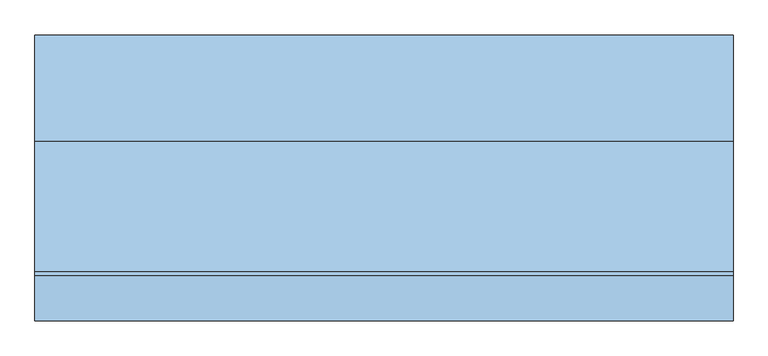
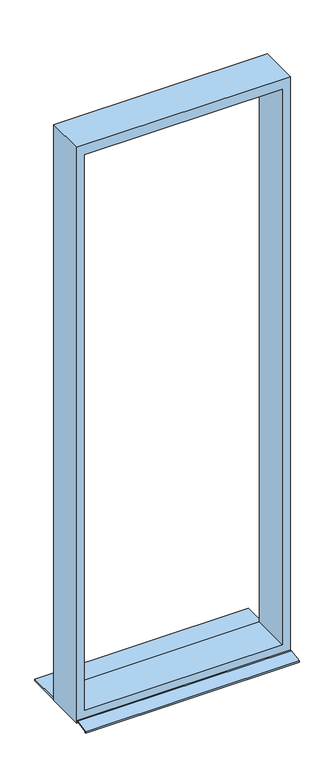
"""IFC4 building model written with IfcOpenShell, lengths in millimetres: window geometry, Fenster - Festverglasung : Feste Verglasung 4.58 x 1.61 2."""

from ifc_helpers import new_model, si_unit, frame, origin, place, context, project, spatial, polyline, outline, extrude, source, transform, mapped, element, save


def window_990d40f6(model_context):
    return source(origin(), model_context, "Body", "SweptSolid", [
        extrude(outline(polyline([(5580.0, 805.0), (5580.0, -805.0), (1000.0, -805.0), (1000.0, 805.0), (5580.0, 805.0)]), holes=[polyline([(5500.0, 745.0), (1080.0, 745.0), (1080.0, -745.0), (5500.0, -745.0), (5500.0, 745.0)])]), frame((0.0, -215.8682116, 0.0), z_axis=(0.0, 1.0, 0.0), x_axis=(0.0, 0.0, 1.0)), (0.0, 0.0, 1.0), 300.0),
        extrude(outline(polyline([(-805.0, 330.0), (805.0, 330.0), (805.0, 84.1317884), (-805.0, 84.1317884), (-805.0, 330.0)])), frame((0.0, 0.0, 1005.0), z_axis=(0.0, 0.0, 1.0), x_axis=(1.0, 0.0, 0.0)), (0.0, 0.0, 1.0), 15.0),
        extrude(outline(polyline([(-225.8903659, 1020.0), (-215.8682116, 1020.0), (-215.8682116, 1018.0), (-225.6922839, 1018.0), (-328.0, 998.3604634), (-328.0, 990.0), (-330.0, 990.0), (-330.0, 1000.0), (-225.8903659, 1020.0)])), frame((-805.0, 0.0, 0.0), z_axis=(1.0, 0.0, 0.0), x_axis=(0.0, 1.0, 0.0)), (0.0, 0.0, 1.0), 1610.0),
    ])


if __name__ == "__main__":
    model = new_model("IFC4")
    model_context = context("Model", 3, world=origin())
    ifc_project = project(units=[si_unit("LENGTHUNIT", "METRE", prefix="MILLI")], contexts=[model_context])
    site = spatial("IfcSite", under=ifc_project)
    building = spatial("IfcBuilding", under=site)
    placement = place(None, origin())
    window_shape = window_990d40f6(model_context)
    element("IfcWindow", 1, ObjectType="Fenster - Festverglasung : Feste Verglasung 4.58 x 1.61 2", at=placement, inside=building, context=model_context, shape_type="MappedRepresentation", body=[
        mapped(window_shape, transform((0.0, 0.0, 0.0), x_axis=(1.0, 0.0, 0.0), y_axis=(0.0, 1.0, 0.0), z_axis=(0.0, 0.0, 1.0))),
    ])
    save(model, "model.ifc")

# Revit data of these elements
# Type "Fenster - Festverglasung : Feste Verglasung 4.58 x 1.61 2"
#   Type Mark = "60"
#   Operation = "SinglePanel"
#   Keynote = "16.05.01"
#   Visual Light Transmittance = 0.9
#   Solar Heat Gain Coefficient = 0.78
#   Rough Width = 1.610 m
#   Rough Height = 4.580 m
#   Heat Transfer Coefficient (U) = 3.6886 W/(m²·K)
#   Rahmentiefe = 0.300 m
#   Rahmenhöhe unten = 0.080 m
#   Höhe oberer  Rahmen = 0.080 m
#   Rahmenbreite = 0.060 m
#   Height = 4.580 m
#   Einbautiefe (von außen) [instance default] = 0.080 m
#   Width = 1.610 m
#   Wall Closure = 3
#   Bild [instance default] = none
#   Glas [instance default] = none
#   Innere Fensterbank [instance default] = none
#   Äußere Fensterbank [instance default] = none
#   Construction Type Id = ""
#   Analytic Construction = (empty or 0)
# Element 1 (IfcWindow, "Fenster - Festverglasung : Feste Verglasung 4.58 x 1.61 2")
#   Einbautiefe (von außen) = 0.084132 m
#   Materials on its faces: "Kunststoff - Weiß", "Holz - Birke"
# Materials
#   "Kunststoff - Weiß": class "Kunststoff", colour RGB 249 249 249, transparency 0, Cost = 0
#   "Holz - Birke": class "Holz", colour RGB 213 164 103, transparency 0, Cost = 0
